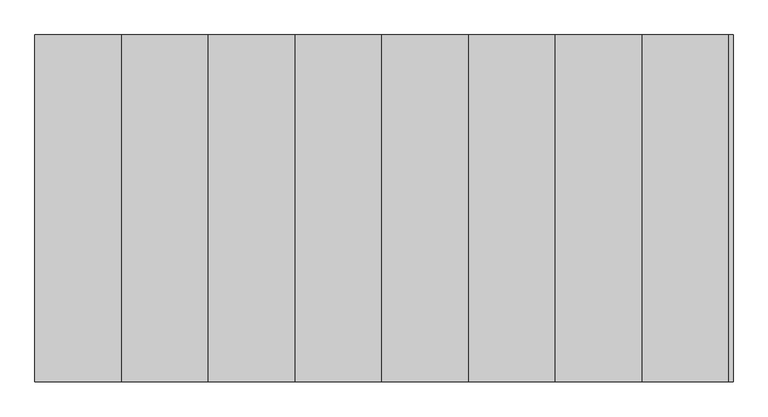
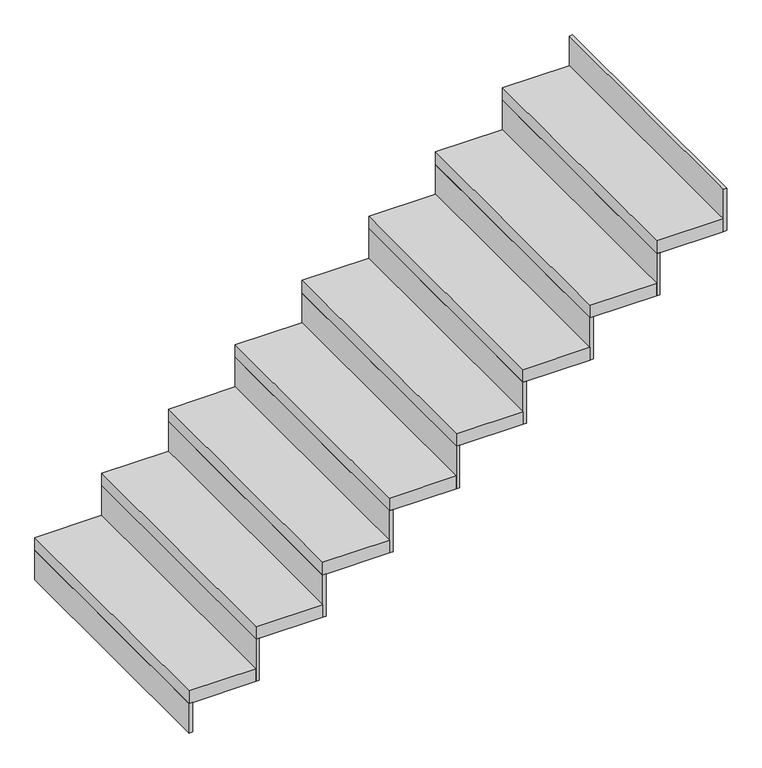
"""IFC4 building model written with IfcOpenShell, lengths in millimetres: stair flight geometry."""

from ifc_helpers import new_model, si_unit, frame, origin, place, context, project, spatial, polyline, outline, extrude, source, transform, mapped, element, save


def stair_flight_022891a7(model_context):
    return source(origin(), model_context, "Body", "SweptSolid", [
        extrude(outline(polyline([(3289.0556606, 2685.7983707), (3276.5556606, 2685.7983707), (3276.5556606, 3685.7983707), (3289.0556606, 3685.7983707), (3289.0556606, 2685.7983707)])), frame((0.0, 0.0, 3300.0), z_axis=(0.0, 0.0, 1.0), x_axis=(1.0, 0.0, 0.0)), (0.0, 0.0, 1.0), 116.6666667),
        extrude(outline(polyline([(3526.5556606, 3685.7983707), (3526.5556606, 2685.7983707), (3276.5556606, 2685.7983707), (3276.5556606, 3685.7983707), (3526.5556606, 3685.7983707)])), frame((0.0, 0.0, 3416.6666667), z_axis=(0.0, 0.0, 1.0), x_axis=(1.0, 0.0, 0.0)), (0.0, 0.0, 1.0), 50.0),
        extrude(outline(polyline([(3539.0556606, 2685.7983707), (3526.5556606, 2685.7983707), (3526.5556606, 3685.7983707), (3539.0556606, 3685.7983707), (3539.0556606, 2685.7983707)])), frame((0.0, 0.0, 3416.6666667), z_axis=(0.0, 0.0, 1.0), x_axis=(1.0, 0.0, 0.0)), (0.0, 0.0, 1.0), 166.6666667),
        extrude(outline(polyline([(3776.5556606, 3685.7983707), (3776.5556606, 2685.7983707), (3526.5556606, 2685.7983707), (3526.5556606, 3685.7983707), (3776.5556606, 3685.7983707)])), frame((0.0, 0.0, 3583.3333333), z_axis=(0.0, 0.0, 1.0), x_axis=(1.0, 0.0, 0.0)), (0.0, 0.0, 1.0), 50.0),
        extrude(outline(polyline([(3789.0556606, 2685.7983707), (3776.5556606, 2685.7983707), (3776.5556606, 3685.7983707), (3789.0556606, 3685.7983707), (3789.0556606, 2685.7983707)])), frame((0.0, 0.0, 3583.3333333), z_axis=(0.0, 0.0, 1.0), x_axis=(1.0, 0.0, 0.0)), (0.0, 0.0, 1.0), 166.6666667),
        extrude(outline(polyline([(4026.5556606, 3685.7983707), (4026.5556606, 2685.7983707), (3776.5556606, 2685.7983707), (3776.5556606, 3685.7983707), (4026.5556606, 3685.7983707)])), frame((0.0, 0.0, 3750.0), z_axis=(0.0, 0.0, 1.0), x_axis=(1.0, 0.0, 0.0)), (0.0, 0.0, 1.0), 50.0),
        extrude(outline(polyline([(4039.0556606, 2685.7983707), (4026.5556606, 2685.7983707), (4026.5556606, 3685.7983707), (4039.0556606, 3685.7983707), (4039.0556606, 2685.7983707)])), frame((0.0, 0.0, 3750.0), z_axis=(0.0, 0.0, 1.0), x_axis=(1.0, 0.0, 0.0)), (0.0, 0.0, 1.0), 166.6666667),
        extrude(outline(polyline([(4276.5556606, 3685.7983707), (4276.5556606, 2685.7983707), (4026.5556606, 2685.7983707), (4026.5556606, 3685.7983707), (4276.5556606, 3685.7983707)])), frame((0.0, 0.0, 3916.6666667), z_axis=(0.0, 0.0, 1.0), x_axis=(1.0, 0.0, 0.0)), (0.0, 0.0, 1.0), 50.0),
        extrude(outline(polyline([(4289.0556606, 2685.7983707), (4276.5556606, 2685.7983707), (4276.5556606, 3685.7983707), (4289.0556606, 3685.7983707), (4289.0556606, 2685.7983707)])), frame((0.0, 0.0, 3916.6666667), z_axis=(0.0, 0.0, 1.0), x_axis=(1.0, 0.0, 0.0)), (0.0, 0.0, 1.0), 166.6666667),
        extrude(outline(polyline([(4526.5556606, 3685.7983707), (4526.5556606, 2685.7983707), (4276.5556606, 2685.7983707), (4276.5556606, 3685.7983707), (4526.5556606, 3685.7983707)])), frame((0.0, 0.0, 4083.3333333), z_axis=(0.0, 0.0, 1.0), x_axis=(1.0, 0.0, 0.0)), (0.0, 0.0, 1.0), 50.0),
        extrude(outline(polyline([(4539.0556606, 2685.7983707), (4526.5556606, 2685.7983707), (4526.5556606, 3685.7983707), (4539.0556606, 3685.7983707), (4539.0556606, 2685.7983707)])), frame((0.0, 0.0, 4083.3333333), z_axis=(0.0, 0.0, 1.0), x_axis=(1.0, 0.0, 0.0)), (0.0, 0.0, 1.0), 166.6666667),
        extrude(outline(polyline([(4776.5556606, 3685.7983707), (4776.5556606, 2685.7983707), (4526.5556606, 2685.7983707), (4526.5556606, 3685.7983707), (4776.5556606, 3685.7983707)])), frame((0.0, 0.0, 4250.0), z_axis=(0.0, 0.0, 1.0), x_axis=(1.0, 0.0, 0.0)), (0.0, 0.0, 1.0), 50.0),
        extrude(outline(polyline([(4789.0556606, 2685.7983707), (4776.5556606, 2685.7983707), (4776.5556606, 3685.7983707), (4789.0556606, 3685.7983707), (4789.0556606, 2685.7983707)])), frame((0.0, 0.0, 4250.0), z_axis=(0.0, 0.0, 1.0), x_axis=(1.0, 0.0, 0.0)), (0.0, 0.0, 1.0), 166.6666667),
        extrude(outline(polyline([(5026.5556606, 3685.7983707), (5026.5556606, 2685.7983707), (4776.5556606, 2685.7983707), (4776.5556606, 3685.7983707), (5026.5556606, 3685.7983707)])), frame((0.0, 0.0, 4416.6666667), z_axis=(0.0, 0.0, 1.0), x_axis=(1.0, 0.0, 0.0)), (0.0, 0.0, 1.0), 50.0),
        extrude(outline(polyline([(5039.0556606, 2685.7983707), (5026.5556606, 2685.7983707), (5026.5556606, 3685.7983707), (5039.0556606, 3685.7983707), (5039.0556606, 2685.7983707)])), frame((0.0, 0.0, 4416.6666667), z_axis=(0.0, 0.0, 1.0), x_axis=(1.0, 0.0, 0.0)), (0.0, 0.0, 1.0), 166.6666667),
        extrude(outline(polyline([(5289.0556606, 2685.7983707), (5276.5556606, 2685.7983707), (5276.5556606, 3685.7983707), (5289.0556606, 3685.7983707), (5289.0556606, 2685.7983707)])), frame((0.0, 0.0, 4583.3333333), z_axis=(0.0, 0.0, 1.0), x_axis=(1.0, 0.0, 0.0)), (0.0, 0.0, 1.0), 166.6666667),
        extrude(outline(polyline([(5276.5556606, 3685.7983707), (5276.5556606, 2685.7983707), (5026.5556606, 2685.7983707), (5026.5556606, 3685.7983707), (5276.5556606, 3685.7983707)])), frame((0.0, 0.0, 4583.3333333), z_axis=(0.0, 0.0, 1.0), x_axis=(1.0, 0.0, 0.0)), (0.0, 0.0, 1.0), 50.0),
    ])


if __name__ == "__main__":
    model = new_model("IFC4")
    model_context = context("Model", 3, world=origin())
    ifc_project = project(units=[si_unit("LENGTHUNIT", "METRE", prefix="MILLI")], contexts=[model_context])
    site = spatial("IfcSite", under=ifc_project)
    building = spatial("IfcBuilding", under=site)
    placement = place(None, origin())
    stair_flight_shape = stair_flight_022891a7(model_context)
    element("IfcStairFlight", 1, at=placement, inside=building, context=model_context, shape_type="MappedRepresentation", body=[
        mapped(stair_flight_shape, transform((0.0, 0.0, 0.0), x_axis=(1.0, 0.0, 0.0), y_axis=(0.0, 1.0, 0.0), z_axis=(0.0, 0.0, 1.0))),
    ])
    save(model, "model.ifc")

# Revit data of these elements
# Project information
#   项目发布日期 = "出图日期"
#   项目状态 = "项目状态"
#   客户姓名 = "所有者"
#   项目地址 = "请在此处输入地址"
#   项目名称 = "项目名称"
#   项目编号 = "项目编号"
